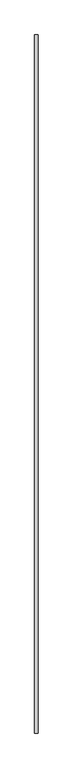
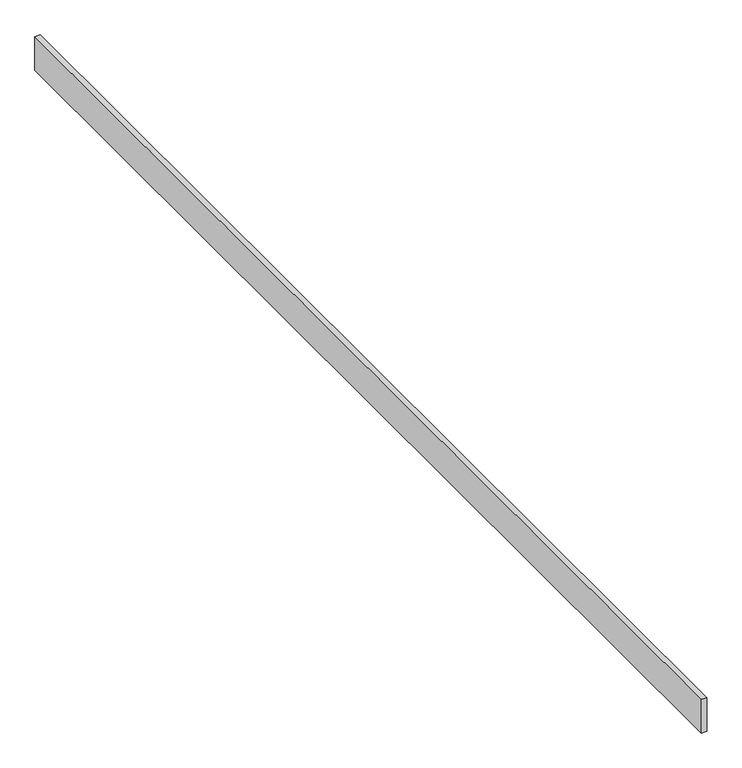
"""IFC4 building model written with IfcOpenShell, lengths in millimetres: proxy geometry, Generic Models 7:Generic Models 1:6:Generic Models 1:6 : Generic Models 7:Generic Models 1:337419:12 : Generic Models 7:Generic Models 1:6:Generic Models 1:6 : Generic Models 7:Generic Models 1:337419:312901."""

from ifc_helpers import new_model, si_unit, frame, origin, place, context, project, spatial, polyline, outline, extrude, source, transform, mapped, element, save


def generic_models_62f418d0(model_context):
    return source(origin(), model_context, "Body", "SweptSolid", [
        extrude(outline(polyline([(667547.3117239, -578051.3663841), (667344.1117239, -578051.3663841), (667344.1117239, -533550.5663841), (667547.3117239, -533550.5663841), (667547.3117239, -578051.3663841)])), frame((0.0, 0.0, -1377.3372439), z_axis=(0.0, 0.0, 1.0), x_axis=(1.0, 0.0, 0.0)), (0.0, 0.0, 1.0), 1377.3372439),
    ])


if __name__ == "__main__":
    model = new_model("IFC4")
    model_context = context("Model", 3, world=origin())
    ifc_project = project(units=[si_unit("LENGTHUNIT", "METRE", prefix="MILLI")], contexts=[model_context])
    site = spatial("IfcSite", under=ifc_project)
    building = spatial("IfcBuilding", under=site)
    placement = place(None, origin())
    generic_models_shape = generic_models_62f418d0(model_context)
    element("IfcBuildingElementProxy", 1, Name="Generic Models 7:Generic Models 1:6:Generic Models 1:6 : Generic Models 7:Generic Models 1:337419:12 : Generic Models 7:Generic Models 1:6:Generic Models 1:6 : Generic Models 7:Generic Models 1:337419:312901", ObjectType="Generic Models 7:Generic Models 1:6:Generic Models 1:6 : Generic Models 7:Generic Models 1:337419:12 : Generic Models 7:Generic Models 1:6:Generic Models 1:6 : Generic Models 7:Generic Models 1:337419:312901", at=placement, inside=building, context=model_context, shape_type="MappedRepresentation", body=[
        mapped(generic_models_shape, transform((0.0, 0.0, 0.0), x_axis=(1.0, 0.0, 0.0), y_axis=(0.0, 1.0, 0.0), z_axis=(0.0, 0.0, 1.0))),
    ])
    save(model, "model.ifc")

# Revit data of these elements
# Type "Generic Models 7:Generic Models 1:6:Generic Models 1:6 : Generic Models 7:Generic Models 1:337419:12 : Generic Models 7:Generic Models 1:6:Generic Models 1:6 : Generic Models 7:Generic Models 1:337419:312901"
#   NameOverride = "Generic Models 7:Generic Models 1:6:Generic Models 1:6 : Generic Models 7:Generic Models 1:337419:312901"
#   ObjectTypeOverride = "Generic Models 1:6 : Generic Models 7:Generic Models 1:337419"
#   Reference = "Generic Models 1"
#   Tag = "312901"
# Element 1 (IfcBuildingElementProxy, "Generic Models 7:Generic Models 1:6:Generic Models 1:6 : Generic Models 7:Generic Models 1:337419:12 : Generic Models 7:Generic Models 1:6:Generic Models 1:6 : Generic Models 7:Generic Models 1:337419:312901")
#   Materials on its faces: "CONCRETE FROST WALL - SEE STRUCT DWGS."
# Materials
#   "CONCRETE FROST WALL - SEE STRUCT DWGS.": class "Concrete", colour RGB 115 116 108, transparency 0, Description = "Lightweight concrete", Cost = 0
